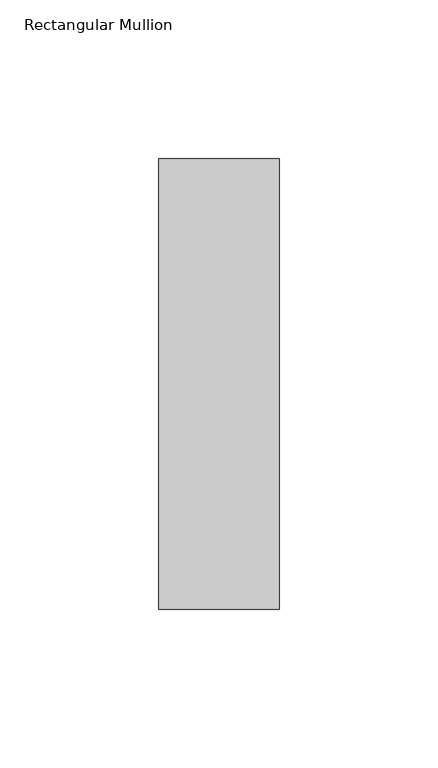
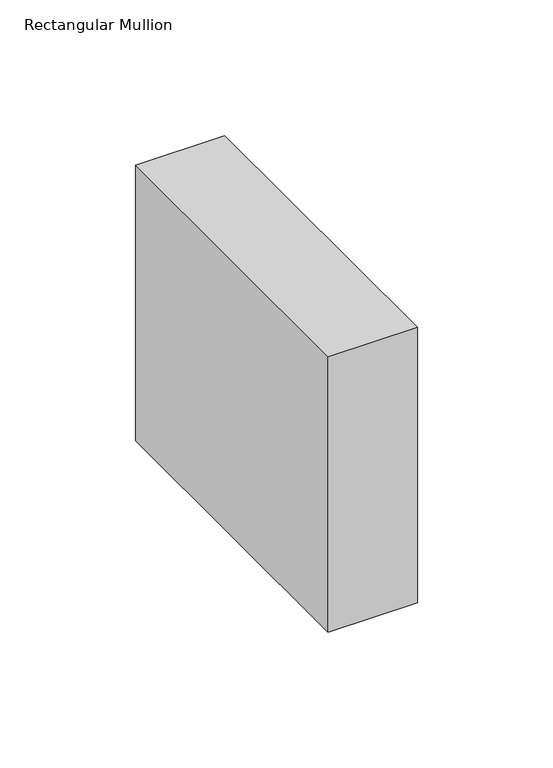
"""IFC4 building model written with IfcOpenShell, lengths in millimetres: member geometry, Rectangular Mullion : NLRS_21_CWM_hsb-regel 38x142_gen_rsf."""

from ifc_helpers import new_model, si_unit, frame, origin, place, context, project, spatial, polyline, outline, extrude, source, transform, mapped, element, save


def rectangular_mullion_21a1eeaa(model_context):
    return source(origin(), model_context, "Body", "SweptSolid", [
        extrude(outline(polyline([(-38.0, -71.0), (-38.0, 71.0), (0.0, 71.0), (0.0, -71.0), (-38.0, -71.0)])), frame((0.0, 0.0, -123.9999997), z_axis=(0.0, 0.0, 1.0), x_axis=(1.0, 0.0, 0.0)), (0.0, 0.0, 1.0), 123.9999997),
    ])


if __name__ == "__main__":
    model = new_model("IFC4")
    model_context = context("Model", 3, world=origin())
    ifc_project = project(units=[si_unit("LENGTHUNIT", "METRE", prefix="MILLI")], contexts=[model_context])
    site = spatial("IfcSite", under=ifc_project)
    building = spatial("IfcBuilding", under=site)
    placement = place(None, origin())
    rectangular_mullion_shape = rectangular_mullion_21a1eeaa(model_context)
    element("IfcMember", 1, ObjectType="Rectangular Mullion : NLRS_21_CWM_hsb-regel 38x142_gen_rsf", at=placement, inside=building, context=model_context, shape_type="MappedRepresentation", body=[
        mapped(rectangular_mullion_shape, transform((0.0, 0.0, 0.0), x_axis=(1.0, 0.0, 0.0), y_axis=(0.0, 1.0, 0.0), z_axis=(0.0, 0.0, 1.0))),
    ])
    save(model, "model.ifc")

# Revit data of these elements
# Type "Rectangular Mullion : NLRS_21_CWM_hsb-regel 38x142_gen_rsf"
#   Export Type to IFC As = "IfcWall"
#   Type IfcGUID = "07M7mRoiH1CR8m_RSKIwpF"
#   Assembly Code = "21.10"
#   built-in parameter 1007322 = 0.465879 (stored number, unit not read)
#   built-in parameter 1007321 = 0.062336 (stored number, unit not read)
#   built-in parameter 1007320 = 0.062336 (stored number, unit not read)
# Element 1 (IfcMember, "Rectangular Mullion : NLRS_21_CWM_hsb-regel 38x142_gen_rsf")
#   Materials on its faces: "NLRS_i2_hout naaldhout vuren_gen_rsf"
# Materials
#   "NLRS_i2_hout naaldhout vuren_gen_rsf": class "I - Hout", colour RGB 234 199 147, transparency 0, Keynote = "i2", Manufacturer = "Revit Standards Foundation", URL = "www.revitstandards.org", Description = "hout vuren", Cost = 0
